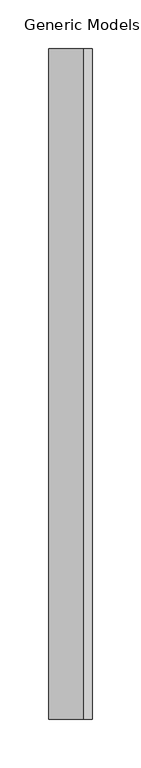
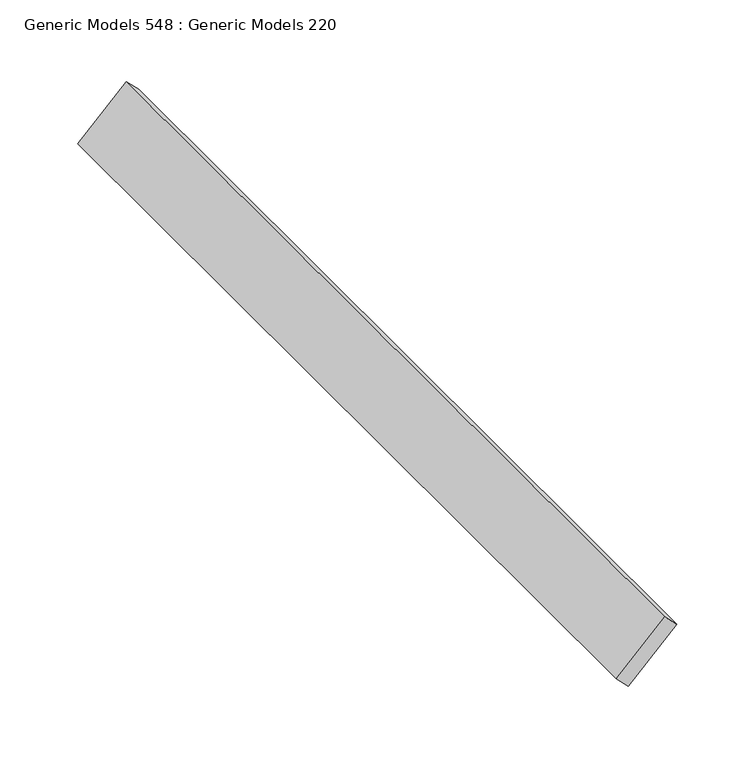
"""IFC4 building model written with IfcOpenShell, lengths in millimetres: proxy geometry, Generic Models 548 : Generic Models 220."""

from ifc_helpers import new_model, si_unit, frame, origin, place, context, project, spatial, polyline, outline, extrude, source, transform, mapped, element, save


def generic_models_548_generic_models_220_158a12c7(model_context):
    return source(origin(), model_context, "Body", "SweptSolid", [
        extrude(outline(polyline([(0.0, -12.7000001), (0.0, 0.0), (690.8142348, 0.0), (690.8142348, -12.7000001), (0.0, -12.7000001)])), frame((7841.3059863, 4539.4872686, 124747.6399101), z_axis=(0.7071067811868034, 0.0, 0.7071067811862918), x_axis=(0.0, -1.0, 0.0)), (0.0, 0.0, 1.0), 50.8),
    ])


if __name__ == "__main__":
    model = new_model("IFC4")
    model_context = context("Model", 3, world=origin())
    ifc_project = project(units=[si_unit("LENGTHUNIT", "METRE", prefix="MILLI")], contexts=[model_context])
    site = spatial("IfcSite", under=ifc_project)
    building = spatial("IfcBuilding", under=site)
    placement = place(None, origin())
    generic_models_548_generic_models_220_shape = generic_models_548_generic_models_220_158a12c7(model_context)
    element("IfcBuildingElementProxy", 1, Name="Generic Models 548 : Generic Models 220", ObjectType="Generic Models 548 : Generic Models 220", at=placement, inside=building, context=model_context, shape_type="MappedRepresentation", body=[
        mapped(generic_models_548_generic_models_220_shape, transform((0.0, 0.0, 0.0), x_axis=(1.0, 0.0, 0.0), y_axis=(0.0, 1.0, 0.0), z_axis=(0.0, 0.0, 1.0))),
    ])
    save(model, "model.ifc")

# Revit data of these elements
# Element 1 (IfcBuildingElementProxy, "Generic Models 548 : Generic Models 220")
#   Materials on its faces: "_WOOD TONE ALUMINUM EXTRUSION SLAT BY KNOTWOOD"
# Materials
#   "_WOOD TONE ALUMINUM EXTRUSION SLAT BY KNOTWOOD": class "Generic", colour RGB 177 130 114, transparency 0, Cost = 0
